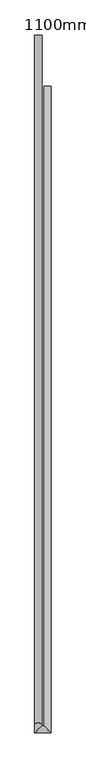
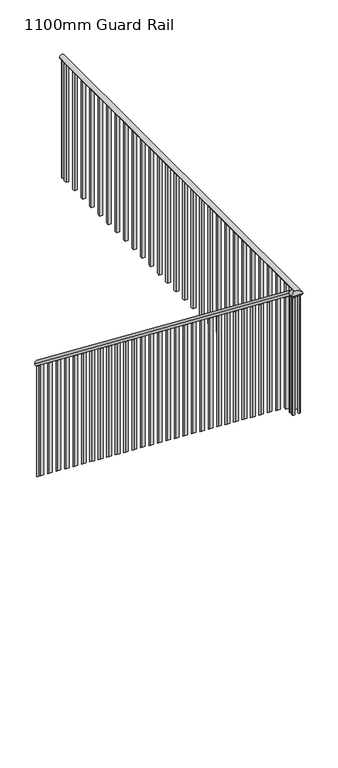
"""IFC4 building model written with IfcOpenShell, lengths in millimetres: railing geometry, 1100mm Guard Rail."""

from ifc_helpers import new_model, si_unit, point, frame, frame_2d, origin, place, context, project, spatial, polyline, circle_curve, ellipse_curve, trimmed, segment, composite_curve, outline, extrude, source, transform, mapped, element, save
from ifc_brep_helpers import plane_surface, cylinder_surface, advanced_brep


def railing_1100mm_guard_rail_56a39491(model_context):
    return source(origin(), model_context, "Body", "SolidModel", [
        advanced_brep(
        [(1386.4, -5975.0, 1268.4468381), (1426.4, -5975.0, 1268.4468381), (1386.4, -9731.8427895, 4180.0), (1426.4, -9731.8427895, 4180.0), (1426.4, -9740.0, 4180.0), (1386.4, -9780.0, 4180.0), (1476.4, -9780.0, 4180.0), (1436.4, -9740.0, 4180.0), (1476.4, -6255.0, 4180.0), (1436.4, -6255.0, 4180.0)],
        [
            (0, 1, ellipse_curve(frame((1406.4, -5975.0, 1268.4468381), z_axis=(0.0, 1.0, 0.0), x_axis=(0.0, 0.0, -0.9999999999999999)), 25.3031619, 20.0)),
            (1, 0, ellipse_curve(frame((1406.4, -5975.0, 1268.4468381), z_axis=(0.0, 1.0, 0.0), x_axis=(0.0, 0.0, -0.9999999999999999)), 25.3031619, 20.0)),
            (0, 2),
            (2, 3, ellipse_curve(frame((1406.4, -9731.8427895, 4180.0), z_axis=(0.0, 0.9461540710093743, -0.32371665683493567), x_axis=(0.0, -0.3237166568349349, -0.9461540710093748)), 21.1382064, 20.0)),
            (3, 1),
            (3, 2, ellipse_curve(frame((1406.4, -9731.8427895, 4180.0), z_axis=(0.0, 0.9461540710093743, -0.32371665683493567), x_axis=(0.0, -0.3237166568349349, -0.9461540710093748)), 21.1382064, 20.0)),
            (4, 5, ellipse_curve(frame((1406.4, -9760.0, 4180.0), z_axis=(0.7071067811865452, -0.7071067811865498, 0.0), x_axis=(-0.7071067811865498, -0.7071067811865451, 0.0)), 28.2842712, 20.0)),
            (5, 6),
            (6, 7, ellipse_curve(frame((1456.4, -9760.0, 4180.0), z_axis=(-0.7071067811865503, -0.7071067811865447, 0.0), x_axis=(-0.7071067811865446, 0.7071067811865503, 0.0)), 28.2842712, 20.0)),
            (7, 4),
            (5, 4, ellipse_curve(frame((1406.4, -9760.0, 4180.0), z_axis=(0.7071067811865452, -0.7071067811865498, 0.0), x_axis=(-0.7071067811865498, -0.7071067811865451, 0.0)), 28.2842712, 20.0)),
            (7, 6, ellipse_curve(frame((1456.4, -9760.0, 4180.0), z_axis=(-0.7071067811865503, -0.7071067811865447, 0.0), x_axis=(-0.7071067811865446, 0.7071067811865503, 0.0)), 28.2842712, 20.0)),
            (8, 9, circle_curve(frame((1456.4, -6255.0, 4180.0), z_axis=(0.0, 1.0, 0.0), x_axis=(-1.0, 0.0, 0.0)), 20.0)),
            (9, 8, circle_curve(frame((1456.4, -6255.0, 4180.0), z_axis=(0.0, 1.0, 0.0), x_axis=(-1.0, 0.0, 0.0)), 20.0)),
            (6, 8),
            (9, 7),
            (2, 5),
            (4, 3),
        ],
        [
            plane_surface(frame((1406.4, -5975.0, 1293.75), z_axis=(0.0, 1.0, 0.0), x_axis=(0.0, 0.0, -1.0))),
            cylinder_surface(frame((1406.4, -5987.2514333, 1277.941699), z_axis=(0.0, 0.7904150521752251, -0.6125716654358381), x_axis=(1.0, 0.0, 0.0)), 20.0),
            cylinder_surface(frame((1406.4, -9760.0, 4180.0), z_axis=(-1.0, 0.0, 0.0), x_axis=(0.0, 1.0, 0.0)), 20.0),
            plane_surface(frame((1456.4, -6255.0, 4200.0), z_axis=(0.0, 1.0, 0.0), x_axis=(0.0, 0.0, 1.0))),
            cylinder_surface(frame((1456.4, -9760.0, 4180.0), z_axis=(0.0, -1.0, 0.0), x_axis=(-1.0, 0.0, 0.0)), 20.0),
            cylinder_surface(frame((1406.4, -9725.0, 4180.0), z_axis=(0.0, 1.0, 0.0), x_axis=(1.0, 0.0, 0.0)), 20.0),
        ],
        [
            (0, [[1, 2]]),
            (1, [[-1, 3, 4, 5]]),
            (1, [[-2, -5, 6, -3]]),
            (2, [[7, 8, 9, 10]]),
            (2, [[11, -10, 12, -8]]),
            (3, [[13, 14]]),
            (4, [[-9, 15, -14, 16]]),
            (4, [[-12, -16, -13, -15]]),
            (5, [[-4, 17, -7, 18]]),
            (5, [[-6, -18, -11, -17]]),
        ],
    ),
        extrude(outline(polyline([(1443.9, -6335.0), (1443.9, -6310.0), (1468.9, -6310.0), (1468.9, -6335.0), (1443.9, -6335.0)])), frame((0.0, 0.0, 3100.0), z_axis=(0.0, 0.0, 1.0), x_axis=(1.0, 0.0, 0.0)), (0.0, 0.0, 1.0), 1060.0),
        extrude(outline(polyline([(1443.9, -6460.0), (1443.9, -6435.0), (1468.9, -6435.0), (1468.9, -6460.0), (1443.9, -6460.0)])), frame((0.0, 0.0, 3100.0), z_axis=(0.0, 0.0, 1.0), x_axis=(1.0, 0.0, 0.0)), (0.0, 0.0, 1.0), 1060.0),
        extrude(outline(polyline([(1443.9, -6585.0), (1443.9, -6560.0), (1468.9, -6560.0), (1468.9, -6585.0), (1443.9, -6585.0)])), frame((0.0, 0.0, 3100.0), z_axis=(0.0, 0.0, 1.0), x_axis=(1.0, 0.0, 0.0)), (0.0, 0.0, 1.0), 1060.0),
        extrude(outline(polyline([(1443.9, -6710.0), (1443.9, -6685.0), (1468.9, -6685.0), (1468.9, -6710.0), (1443.9, -6710.0)])), frame((0.0, 0.0, 3100.0), z_axis=(0.0, 0.0, 1.0), x_axis=(1.0, 0.0, 0.0)), (0.0, 0.0, 1.0), 1060.0),
        extrude(outline(polyline([(1443.9, -6835.0), (1443.9, -6810.0), (1468.9, -6810.0), (1468.9, -6835.0), (1443.9, -6835.0)])), frame((0.0, 0.0, 3100.0), z_axis=(0.0, 0.0, 1.0), x_axis=(1.0, 0.0, 0.0)), (0.0, 0.0, 1.0), 1060.0),
        extrude(outline(polyline([(1443.9, -6960.0), (1443.9, -6935.0), (1468.9, -6935.0), (1468.9, -6960.0), (1443.9, -6960.0)])), frame((0.0, 0.0, 3100.0), z_axis=(0.0, 0.0, 1.0), x_axis=(1.0, 0.0, 0.0)), (0.0, 0.0, 1.0), 1060.0),
        extrude(outline(polyline([(1443.9, -7085.0), (1443.9, -7060.0), (1468.9, -7060.0), (1468.9, -7085.0), (1443.9, -7085.0)])), frame((0.0, 0.0, 3100.0), z_axis=(0.0, 0.0, 1.0), x_axis=(1.0, 0.0, 0.0)), (0.0, 0.0, 1.0), 1060.0),
        extrude(outline(polyline([(1443.9, -7210.0), (1443.9, -7185.0), (1468.9, -7185.0), (1468.9, -7210.0), (1443.9, -7210.0)])), frame((0.0, 0.0, 3100.0), z_axis=(0.0, 0.0, 1.0), x_axis=(1.0, 0.0, 0.0)), (0.0, 0.0, 1.0), 1060.0),
        extrude(outline(polyline([(1443.9, -7335.0), (1443.9, -7310.0), (1468.9, -7310.0), (1468.9, -7335.0), (1443.9, -7335.0)])), frame((0.0, 0.0, 3100.0), z_axis=(0.0, 0.0, 1.0), x_axis=(1.0, 0.0, 0.0)), (0.0, 0.0, 1.0), 1060.0),
        extrude(outline(polyline([(1443.9, -7460.0), (1443.9, -7435.0), (1468.9, -7435.0), (1468.9, -7460.0), (1443.9, -7460.0)])), frame((0.0, 0.0, 3100.0), z_axis=(0.0, 0.0, 1.0), x_axis=(1.0, 0.0, 0.0)), (0.0, 0.0, 1.0), 1060.0),
        extrude(outline(polyline([(1443.9, -7585.0), (1443.9, -7560.0), (1468.9, -7560.0), (1468.9, -7585.0), (1443.9, -7585.0)])), frame((0.0, 0.0, 3100.0), z_axis=(0.0, 0.0, 1.0), x_axis=(1.0, 0.0, 0.0)), (0.0, 0.0, 1.0), 1060.0),
        extrude(outline(polyline([(1443.9, -7710.0), (1443.9, -7685.0), (1468.9, -7685.0), (1468.9, -7710.0), (1443.9, -7710.0)])), frame((0.0, 0.0, 3100.0), z_axis=(0.0, 0.0, 1.0), x_axis=(1.0, 0.0, 0.0)), (0.0, 0.0, 1.0), 1060.0),
        extrude(outline(polyline([(1443.9, -7835.0), (1443.9, -7810.0), (1468.9, -7810.0), (1468.9, -7835.0), (1443.9, -7835.0)])), frame((0.0, 0.0, 3100.0), z_axis=(0.0, 0.0, 1.0), x_axis=(1.0, 0.0, 0.0)), (0.0, 0.0, 1.0), 1060.0),
        extrude(outline(polyline([(1443.9, -7960.0), (1443.9, -7935.0), (1468.9, -7935.0), (1468.9, -7960.0), (1443.9, -7960.0)])), frame((0.0, 0.0, 3100.0), z_axis=(0.0, 0.0, 1.0), x_axis=(1.0, 0.0, 0.0)), (0.0, 0.0, 1.0), 1060.0),
        extrude(outline(polyline([(1443.9, -8085.0), (1443.9, -8060.0), (1468.9, -8060.0), (1468.9, -8085.0), (1443.9, -8085.0)])), frame((0.0, 0.0, 3100.0), z_axis=(0.0, 0.0, 1.0), x_axis=(1.0, 0.0, 0.0)), (0.0, 0.0, 1.0), 1060.0),
        extrude(outline(polyline([(1443.9, -8210.0), (1443.9, -8185.0), (1468.9, -8185.0), (1468.9, -8210.0), (1443.9, -8210.0)])), frame((0.0, 0.0, 3100.0), z_axis=(0.0, 0.0, 1.0), x_axis=(1.0, 0.0, 0.0)), (0.0, 0.0, 1.0), 1060.0),
        extrude(outline(polyline([(1443.9, -8335.0), (1443.9, -8310.0), (1468.9, -8310.0), (1468.9, -8335.0), (1443.9, -8335.0)])), frame((0.0, 0.0, 3100.0), z_axis=(0.0, 0.0, 1.0), x_axis=(1.0, 0.0, 0.0)), (0.0, 0.0, 1.0), 1060.0),
        extrude(outline(polyline([(1443.9, -8460.0), (1443.9, -8435.0), (1468.9, -8435.0), (1468.9, -8460.0), (1443.9, -8460.0)])), frame((0.0, 0.0, 3100.0), z_axis=(0.0, 0.0, 1.0), x_axis=(1.0, 0.0, 0.0)), (0.0, 0.0, 1.0), 1060.0),
        extrude(outline(polyline([(1443.9, -8585.0), (1443.9, -8560.0), (1468.9, -8560.0), (1468.9, -8585.0), (1443.9, -8585.0)])), frame((0.0, 0.0, 3100.0), z_axis=(0.0, 0.0, 1.0), x_axis=(1.0, 0.0, 0.0)), (0.0, 0.0, 1.0), 1060.0),
        extrude(outline(polyline([(1443.9, -8710.0), (1443.9, -8685.0), (1468.9, -8685.0), (1468.9, -8710.0), (1443.9, -8710.0)])), frame((0.0, 0.0, 3100.0), z_axis=(0.0, 0.0, 1.0), x_axis=(1.0, 0.0, 0.0)), (0.0, 0.0, 1.0), 1060.0),
        extrude(outline(polyline([(1443.9, -8835.0), (1443.9, -8810.0), (1468.9, -8810.0), (1468.9, -8835.0), (1443.9, -8835.0)])), frame((0.0, 0.0, 3100.0), z_axis=(0.0, 0.0, 1.0), x_axis=(1.0, 0.0, 0.0)), (0.0, 0.0, 1.0), 1060.0),
        extrude(outline(polyline([(1443.9, -8960.0), (1443.9, -8935.0), (1468.9, -8935.0), (1468.9, -8960.0), (1443.9, -8960.0)])), frame((0.0, 0.0, 3100.0), z_axis=(0.0, 0.0, 1.0), x_axis=(1.0, 0.0, 0.0)), (0.0, 0.0, 1.0), 1060.0),
        extrude(outline(polyline([(1443.9, -9085.0), (1443.9, -9060.0), (1468.9, -9060.0), (1468.9, -9085.0), (1443.9, -9085.0)])), frame((0.0, 0.0, 3100.0), z_axis=(0.0, 0.0, 1.0), x_axis=(1.0, 0.0, 0.0)), (0.0, 0.0, 1.0), 1060.0),
        extrude(outline(polyline([(1443.9, -9210.0), (1443.9, -9185.0), (1468.9, -9185.0), (1468.9, -9210.0), (1443.9, -9210.0)])), frame((0.0, 0.0, 3100.0), z_axis=(0.0, 0.0, 1.0), x_axis=(1.0, 0.0, 0.0)), (0.0, 0.0, 1.0), 1060.0),
        extrude(outline(polyline([(1443.9, -9335.0), (1443.9, -9310.0), (1468.9, -9310.0), (1468.9, -9335.0), (1443.9, -9335.0)])), frame((0.0, 0.0, 3100.0), z_axis=(0.0, 0.0, 1.0), x_axis=(1.0, 0.0, 0.0)), (0.0, 0.0, 1.0), 1060.0),
        extrude(outline(polyline([(1443.9, -9460.0), (1443.9, -9435.0), (1468.9, -9435.0), (1468.9, -9460.0), (1443.9, -9460.0)])), frame((0.0, 0.0, 3100.0), z_axis=(0.0, 0.0, 1.0), x_axis=(1.0, 0.0, 0.0)), (0.0, 0.0, 1.0), 1060.0),
        extrude(outline(polyline([(1443.9, -9585.0), (1443.9, -9560.0), (1468.9, -9560.0), (1468.9, -9585.0), (1443.9, -9585.0)])), frame((0.0, 0.0, 3100.0), z_axis=(0.0, 0.0, 1.0), x_axis=(1.0, 0.0, 0.0)), (0.0, 0.0, 1.0), 1060.0),
        extrude(outline(polyline([(1443.9, -9710.0), (1443.9, -9685.0), (1468.9, -9685.0), (1468.9, -9710.0), (1443.9, -9710.0)])), frame((0.0, 0.0, 3100.0), z_axis=(0.0, 0.0, 1.0), x_axis=(1.0, 0.0, 0.0)), (0.0, 0.0, 1.0), 1060.0),
        extrude(outline(polyline([(-9650.0, 3100.0), (-9675.0, 3100.0), (-9675.0, 4110.6436763), (-9650.0, 4091.2686763), (-9650.0, 3100.0)])), frame((1393.9, 0.0, 0.0), z_axis=(1.0, 0.0, 0.0), x_axis=(0.0, 1.0, 0.0)), (0.0, 0.0, 1.0), 25.0),
        extrude(outline(polyline([(-9525.0, 2997.571707), (-9550.0, 3016.946707), (-9550.0, 4013.7686763), (-9525.0, 3994.3936763), (-9525.0, 2997.571707)])), frame((1393.9, 0.0, 0.0), z_axis=(1.0, 0.0, 0.0), x_axis=(0.0, 1.0, 0.0)), (0.0, 0.0, 1.0), 25.0),
        extrude(outline(polyline([(-9400.0, 2900.696707), (-9425.0, 2920.071707), (-9425.0, 3916.8936763), (-9400.0, 3897.5186763), (-9400.0, 2900.696707)])), frame((1393.9, 0.0, 0.0), z_axis=(1.0, 0.0, 0.0), x_axis=(0.0, 1.0, 0.0)), (0.0, 0.0, 1.0), 25.0),
        extrude(outline(polyline([(-9275.0, 2803.821707), (-9300.0, 2823.196707), (-9300.0, 3820.0186763), (-9275.0, 3800.6436763), (-9275.0, 2803.821707)])), frame((1393.9, 0.0, 0.0), z_axis=(1.0, 0.0, 0.0), x_axis=(0.0, 1.0, 0.0)), (0.0, 0.0, 1.0), 25.0),
        extrude(outline(polyline([(-9150.0, 2706.946707), (-9175.0, 2726.321707), (-9175.0, 3723.1436763), (-9150.0, 3703.7686763), (-9150.0, 2706.946707)])), frame((1393.9, 0.0, 0.0), z_axis=(1.0, 0.0, 0.0), x_axis=(0.0, 1.0, 0.0)), (0.0, 0.0, 1.0), 25.0),
        extrude(outline(polyline([(-9025.0, 2610.071707), (-9050.0, 2629.446707), (-9050.0, 3626.2686763), (-9025.0, 3606.8936763), (-9025.0, 2610.071707)])), frame((1393.9, 0.0, 0.0), z_axis=(1.0, 0.0, 0.0), x_axis=(0.0, 1.0, 0.0)), (0.0, 0.0, 1.0), 25.0),
        extrude(outline(polyline([(-8900.0, 2513.196707), (-8925.0, 2532.571707), (-8925.0, 3529.3936763), (-8900.0, 3510.0186763), (-8900.0, 2513.196707)])), frame((1393.9, 0.0, 0.0), z_axis=(1.0, 0.0, 0.0), x_axis=(0.0, 1.0, 0.0)), (0.0, 0.0, 1.0), 25.0),
        extrude(outline(polyline([(-8775.0, 2416.321707), (-8800.0, 2435.696707), (-8800.0, 3432.5186763), (-8775.0, 3413.1436763), (-8775.0, 2416.321707)])), frame((1393.9, 0.0, 0.0), z_axis=(1.0, 0.0, 0.0), x_axis=(0.0, 1.0, 0.0)), (0.0, 0.0, 1.0), 25.0),
        extrude(outline(polyline([(-8650.0, 2319.446707), (-8675.0, 2338.821707), (-8675.0, 3335.6436763), (-8650.0, 3316.2686763), (-8650.0, 2319.446707)])), frame((1393.9, 0.0, 0.0), z_axis=(1.0, 0.0, 0.0), x_axis=(0.0, 1.0, 0.0)), (0.0, 0.0, 1.0), 25.0),
        extrude(outline(polyline([(-8525.0, 2222.571707), (-8550.0, 2241.946707), (-8550.0, 3238.7686763), (-8525.0, 3219.3936763), (-8525.0, 2222.571707)])), frame((1393.9, 0.0, 0.0), z_axis=(1.0, 0.0, 0.0), x_axis=(0.0, 1.0, 0.0)), (0.0, 0.0, 1.0), 25.0),
        extrude(outline(polyline([(-8400.0, 2125.696707), (-8425.0, 2145.071707), (-8425.0, 3141.8936763), (-8400.0, 3122.5186763), (-8400.0, 2125.696707)])), frame((1393.9, 0.0, 0.0), z_axis=(1.0, 0.0, 0.0), x_axis=(0.0, 1.0, 0.0)), (0.0, 0.0, 1.0), 25.0),
        extrude(outline(polyline([(-8275.0, 2028.821707), (-8300.0, 2048.196707), (-8300.0, 3045.0186763), (-8275.0, 3025.6436763), (-8275.0, 2028.821707)])), frame((1393.9, 0.0, 0.0), z_axis=(1.0, 0.0, 0.0), x_axis=(0.0, 1.0, 0.0)), (0.0, 0.0, 1.0), 25.0),
        extrude(outline(polyline([(-8150.0, 1931.946707), (-8175.0, 1951.321707), (-8175.0, 2948.1436763), (-8150.0, 2928.7686763), (-8150.0, 1931.946707)])), frame((1393.9, 0.0, 0.0), z_axis=(1.0, 0.0, 0.0), x_axis=(0.0, 1.0, 0.0)), (0.0, 0.0, 1.0), 25.0),
        extrude(outline(polyline([(-8025.0, 1835.071707), (-8050.0, 1854.446707), (-8050.0, 2851.2686763), (-8025.0, 2831.8936763), (-8025.0, 1835.071707)])), frame((1393.9, 0.0, 0.0), z_axis=(1.0, 0.0, 0.0), x_axis=(0.0, 1.0, 0.0)), (0.0, 0.0, 1.0), 25.0),
        extrude(outline(polyline([(-7900.0, 1738.196707), (-7925.0, 1757.571707), (-7925.0, 2754.3936763), (-7900.0, 2735.0186763), (-7900.0, 1738.196707)])), frame((1393.9, 0.0, 0.0), z_axis=(1.0, 0.0, 0.0), x_axis=(0.0, 1.0, 0.0)), (0.0, 0.0, 1.0), 25.0),
        extrude(outline(polyline([(-7775.0, 1641.321707), (-7800.0, 1660.696707), (-7800.0, 2657.5186763), (-7775.0, 2638.1436763), (-7775.0, 1641.321707)])), frame((1393.9, 0.0, 0.0), z_axis=(1.0, 0.0, 0.0), x_axis=(0.0, 1.0, 0.0)), (0.0, 0.0, 1.0), 25.0),
        extrude(outline(polyline([(-7650.0, 1544.446707), (-7675.0, 1563.821707), (-7675.0, 2560.6436763), (-7650.0, 2541.2686763), (-7650.0, 1544.446707)])), frame((1393.9, 0.0, 0.0), z_axis=(1.0, 0.0, 0.0), x_axis=(0.0, 1.0, 0.0)), (0.0, 0.0, 1.0), 25.0),
        extrude(outline(polyline([(-7525.0, 1447.571707), (-7550.0, 1466.946707), (-7550.0, 2463.7686763), (-7525.0, 2444.3936763), (-7525.0, 1447.571707)])), frame((1393.9, 0.0, 0.0), z_axis=(1.0, 0.0, 0.0), x_axis=(0.0, 1.0, 0.0)), (0.0, 0.0, 1.0), 25.0),
        extrude(outline(polyline([(-7400.0, 1350.696707), (-7425.0, 1370.071707), (-7425.0, 2366.8936763), (-7400.0, 2347.5186763), (-7400.0, 1350.696707)])), frame((1393.9, 0.0, 0.0), z_axis=(1.0, 0.0, 0.0), x_axis=(0.0, 1.0, 0.0)), (0.0, 0.0, 1.0), 25.0),
        extrude(outline(polyline([(-7275.0, 1253.821707), (-7300.0, 1273.196707), (-7300.0, 2270.0186763), (-7275.0, 2250.6436763), (-7275.0, 1253.821707)])), frame((1393.9, 0.0, 0.0), z_axis=(1.0, 0.0, 0.0), x_axis=(0.0, 1.0, 0.0)), (0.0, 0.0, 1.0), 25.0),
        extrude(outline(polyline([(-7150.0, 1156.946707), (-7175.0, 1176.321707), (-7175.0, 2173.1436763), (-7150.0, 2153.7686763), (-7150.0, 1156.946707)])), frame((1393.9, 0.0, 0.0), z_axis=(1.0, 0.0, 0.0), x_axis=(0.0, 1.0, 0.0)), (0.0, 0.0, 1.0), 25.0),
        extrude(outline(polyline([(-7025.0, 1060.071707), (-7050.0, 1079.446707), (-7050.0, 2076.2686763), (-7025.0, 2056.8936763), (-7025.0, 1060.071707)])), frame((1393.9, 0.0, 0.0), z_axis=(1.0, 0.0, 0.0), x_axis=(0.0, 1.0, 0.0)), (0.0, 0.0, 1.0), 25.0),
        extrude(outline(polyline([(-6900.0, 963.196707), (-6925.0, 982.571707), (-6925.0, 1979.3936763), (-6900.0, 1960.0186763), (-6900.0, 963.196707)])), frame((1393.9, 0.0, 0.0), z_axis=(1.0, 0.0, 0.0), x_axis=(0.0, 1.0, 0.0)), (0.0, 0.0, 1.0), 25.0),
        extrude(outline(polyline([(-6775.0, 866.321707), (-6800.0, 885.696707), (-6800.0, 1882.5186763), (-6775.0, 1863.1436763), (-6775.0, 866.321707)])), frame((1393.9, 0.0, 0.0), z_axis=(1.0, 0.0, 0.0), x_axis=(0.0, 1.0, 0.0)), (0.0, 0.0, 1.0), 25.0),
        extrude(outline(polyline([(-6650.0, 769.446707), (-6675.0, 788.821707), (-6675.0, 1785.6436763), (-6650.0, 1766.2686763), (-6650.0, 769.446707)])), frame((1393.9, 0.0, 0.0), z_axis=(1.0, 0.0, 0.0), x_axis=(0.0, 1.0, 0.0)), (0.0, 0.0, 1.0), 25.0),
        extrude(outline(polyline([(-6525.0, 672.571707), (-6550.0, 691.946707), (-6550.0, 1688.7686763), (-6525.0, 1669.3936763), (-6525.0, 672.571707)])), frame((1393.9, 0.0, 0.0), z_axis=(1.0, 0.0, 0.0), x_axis=(0.0, 1.0, 0.0)), (0.0, 0.0, 1.0), 25.0),
        extrude(outline(polyline([(-6400.0, 575.696707), (-6425.0, 595.071707), (-6425.0, 1591.8936763), (-6400.0, 1572.5186763), (-6400.0, 575.696707)])), frame((1393.9, 0.0, 0.0), z_axis=(1.0, 0.0, 0.0), x_axis=(0.0, 1.0, 0.0)), (0.0, 0.0, 1.0), 25.0),
        extrude(outline(polyline([(-6275.0, 478.821707), (-6300.0, 498.196707), (-6300.0, 1495.0186763), (-6275.0, 1475.6436763), (-6275.0, 478.821707)])), frame((1393.9, 0.0, 0.0), z_axis=(1.0, 0.0, 0.0), x_axis=(0.0, 1.0, 0.0)), (0.0, 0.0, 1.0), 25.0),
        extrude(outline(polyline([(-6150.0, 381.946707), (-6175.0, 401.321707), (-6175.0, 1398.1436763), (-6150.0, 1378.7686763), (-6150.0, 381.946707)])), frame((1393.9, 0.0, 0.0), z_axis=(1.0, 0.0, 0.0), x_axis=(0.0, 1.0, 0.0)), (0.0, 0.0, 1.0), 25.0),
        extrude(outline(polyline([(-6025.0, 285.071707), (-6050.0, 304.446707), (-6050.0, 1301.2686763), (-6025.0, 1281.8936763), (-6025.0, 285.071707)])), frame((1393.9, 0.0, 0.0), z_axis=(1.0, 0.0, 0.0), x_axis=(0.0, 1.0, 0.0)), (0.0, 0.0, 1.0), 25.0),
        extrude(outline(composite_curve([segment(trimmed(circle_curve(frame_2d((1456.4, -9760.0)), 10.0), [point((1456.4, -9770.0))], [point((1456.4, -9750.0))], False, "CARTESIAN"), True, "CONTINUOUS"), segment(trimmed(circle_curve(frame_2d((1456.4, -9760.0)), 10.0), [point((1456.4, -9750.0))], [point((1456.4, -9770.0))], False, "CARTESIAN"), True, "CONTINUOUS")], self_intersect=False)), frame((0.0, 0.0, 3100.0), z_axis=(0.0, 0.0, 1.0), x_axis=(1.0, 0.0, 0.0)), (0.0, 0.0, 1.0), 1060.0),
        extrude(outline(composite_curve([segment(trimmed(circle_curve(frame_2d((1406.4, -9760.0)), 10.0), [point((1396.4, -9760.0))], [point((1416.4, -9760.0))], False, "CARTESIAN"), True, "CONTINUOUS"), segment(trimmed(circle_curve(frame_2d((1406.4, -9760.0)), 10.0), [point((1416.4, -9760.0))], [point((1396.4, -9760.0))], False, "CARTESIAN"), True, "CONTINUOUS")], self_intersect=False)), frame((0.0, 0.0, 3100.0), z_axis=(0.0, 0.0, 1.0), x_axis=(1.0, 0.0, 0.0)), (0.0, 0.0, 1.0), 1060.0),
        extrude(outline(composite_curve([segment(trimmed(circle_curve(frame_2d((1406.4, -9725.0)), 10.0), [point((1396.4, -9725.0))], [point((1416.4, -9725.0))], False, "CARTESIAN"), True, "CONTINUOUS"), segment(trimmed(circle_curve(frame_2d((1406.4, -9725.0)), 10.0), [point((1416.4, -9725.0))], [point((1396.4, -9725.0))], False, "CARTESIAN"), True, "CONTINUOUS")], self_intersect=False)), frame((0.0, 0.0, 3100.0), z_axis=(0.0, 0.0, 1.0), x_axis=(1.0, 0.0, 0.0)), (0.0, 0.0, 1.0), 1060.0),
        extrude(outline(composite_curve([segment(trimmed(circle_curve(frame_2d((1456.4, -6267.5)), 10.0), [point((1466.4, -6267.5))], [point((1446.4, -6267.5))], False, "CARTESIAN"), True, "CONTINUOUS"), segment(trimmed(circle_curve(frame_2d((1456.4, -6267.5)), 10.0), [point((1446.4, -6267.5))], [point((1466.4, -6267.5))], False, "CARTESIAN"), True, "CONTINUOUS")], self_intersect=False)), frame((0.0, 0.0, 3100.0), z_axis=(0.0, 0.0, 1.0), x_axis=(1.0, 0.0, 0.0)), (0.0, 0.0, 1.0), 1060.0),
        advanced_brep(
        [(1416.4, -5987.5, 1252.8311763), (1396.4, -5987.5, 1252.8311763), (1396.4, -5987.5, 256.009207), (1416.4, -5987.5, 256.009207)],
        [
            (0, 1, ellipse_curve(frame((1406.4, -5987.5, 1252.8311763), z_axis=(0.0, -0.6125716654358373, -0.7904150521752257), x_axis=(0.0, -0.7904150521752258, 0.6125716654358372)), 12.6515809, 10.0)),
            (1, 2),
            (2, 3, ellipse_curve(frame((1406.4, -5987.5, 256.009207), z_axis=(0.0, 0.6125716654358382, 0.790415052175225), x_axis=(0.0, -0.790415052175225, 0.612571665435838)), 12.6515809, 10.0)),
            (3, 0),
            (3, 2, ellipse_curve(frame((1406.4, -5987.5, 256.009207), z_axis=(0.0, 0.6125716654358382, 0.790415052175225), x_axis=(0.0, -0.790415052175225, 0.612571665435838)), 12.6515809, 10.0)),
            (1, 0, ellipse_curve(frame((1406.4, -5987.5, 1252.8311763), z_axis=(0.0, -0.6125716654358373, -0.7904150521752257), x_axis=(0.0, -0.7904150521752258, 0.6125716654358372)), 12.6515809, 10.0)),
        ],
        [
            cylinder_surface(frame((1406.4, -5987.5, 156.009207), z_axis=(0.0, 0.0, 1.0), x_axis=(-1.0, 0.0, 0.0)), 10.0),
            plane_surface(frame((1386.4, -6007.5, 1268.3311763), z_axis=(0.0, 0.6125716654358373, 0.7904150521752257), x_axis=(1.0, 0.0, 0.0))),
            plane_surface(frame((1386.4, -5967.5, 240.509207), z_axis=(0.0, -0.6125716654358382, -0.790415052175225), x_axis=(1.0, 0.0, 0.0))),
        ],
        [
            (0, [[1, 2, 3, 4]]),
            (0, [[5, -2, 6, -4]]),
            (1, [[-6, -1]]),
            (2, [[-5, -3]]),
        ],
    ),
    ])


if __name__ == "__main__":
    model = new_model("IFC4")
    model_context = context("Model", 3, world=origin())
    ifc_project = project(units=[si_unit("LENGTHUNIT", "METRE", prefix="MILLI")], contexts=[model_context])
    site = spatial("IfcSite", under=ifc_project)
    building = spatial("IfcBuilding", under=site)
    placement = place(None, origin())
    railing_1100mm_guard_rail_shape = railing_1100mm_guard_rail_56a39491(model_context)
    element("IfcRailing", 1, ObjectType="1100mm Guard Rail", at=placement, inside=building, context=model_context, shape_type="MappedRepresentation", body=[
        mapped(railing_1100mm_guard_rail_shape, transform((0.0, 0.0, 0.0), x_axis=(1.0, 0.0, 0.0), y_axis=(0.0, 1.0, 0.0), z_axis=(0.0, 0.0, 1.0))),
    ])
    save(model, "model.ifc")
